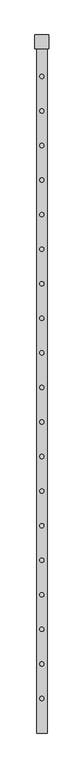
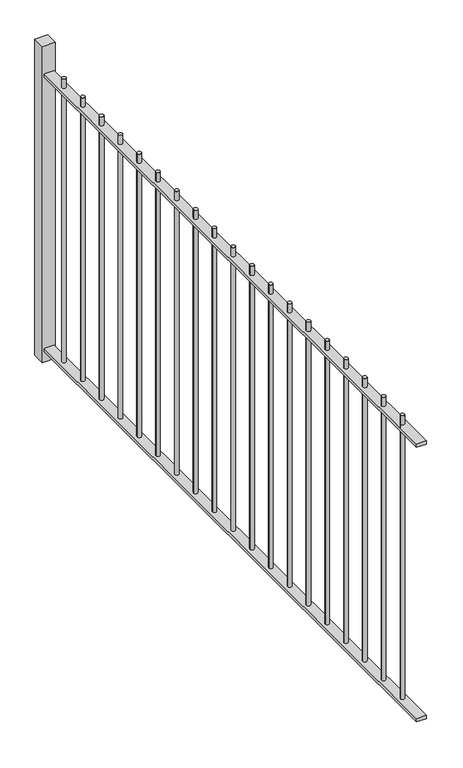
"""IFC4 building model written with IfcOpenShell, lengths in millimetres: railing geometry."""

import ifcopenshell
import ifcopenshell.guid

model = None  # the IFC model being written
_history = None  # IfcOwnerHistory: only IFC2X3 demands one
_inside = {}  # id of a spatial element -> (the spatial element, [elements in it])
_under = {}  # id of a project, library or spatial element -> (it, [spatial elements below it])
_declared = {}  # id of a project -> (the project, [libraries it declares])
_typed = {}  # id of a type object -> (the type object, [elements of that type])
_made_of = {}  # id of a material, layer set ... -> (it, [elements and type objects made of it])


def new_model(schema):
    """Start an empty IFC model of exactly this schema.

    Asked for "IFC4X3", IfcOpenShell would pick the latest addendum, in which some entities
    have other attributes; the version numbers below select the first issue.
    IFC2X3 requires an IfcOwnerHistory on every rooted entity: one is made here for all.
    """
    global model, _history
    if schema == "IFC4X3":
        model = ifcopenshell.file(schema_version=(4, 3, 0, 0))
    else:
        model = ifcopenshell.file(schema=schema)
    _inside.clear()
    _under.clear()
    _declared.clear()
    _typed.clear()
    _made_of.clear()
    _history = None
    if model.schema == "IFC2X3":
        org = make("IfcOrganization", Name="unknown")
        user = make(
            "IfcPersonAndOrganization",
            ThePerson=make("IfcPerson", FamilyName="unknown"),
            TheOrganization=org,
        )
        app = make(
            "IfcApplication",
            ApplicationDeveloper=org,
            Version="unknown",
            ApplicationFullName="unknown",
            ApplicationIdentifier="unknown",
        )
        _history = make(
            "IfcOwnerHistory",
            OwningUser=user,
            OwningApplication=app,
            ChangeAction="ADDED",
            CreationDate=0,
        )
    return model


def make(cls, **values):
    """One entity of the class cls with the attributes given. An attribute that is None is left unset."""
    return model.create_entity(
        cls, **{name: value for name, value in values.items() if value is not None}
    )


def rooted(cls, **values):
    """An entity with a GlobalId (a new one), such as an element, a storey or a relation."""
    return make(cls, GlobalId=ifcopenshell.guid.new(), OwnerHistory=_history, **values)


def si_unit(unit_type, name, prefix=None):
    """IfcSIUnit, for example si_unit("LENGTHUNIT", "METRE", prefix="MILLI")."""
    return make("IfcSIUnit", UnitType=unit_type, Prefix=prefix, Name=name)


def assignment(units):
    """IfcUnitAssignment: the units of a project."""
    return None if units is None else make("IfcUnitAssignment", Units=units)


def point(xyz):
    """IfcCartesianPoint."""
    return None if xyz is None else make("IfcCartesianPoint", Coordinates=xyz)


def direction(xyz):
    """IfcDirection."""
    return None if xyz is None else make("IfcDirection", DirectionRatios=xyz)


def frame(location, z_axis=None, x_axis=None):
    """IfcAxis2Placement3D, a coordinate frame: its origin and axes. An axis left out is left unset."""
    return make(
        "IfcAxis2Placement3D",
        Location=point(location),
        Axis=direction(z_axis),
        RefDirection=direction(x_axis),
    )


def frame_2d(location, x_axis=None):
    """IfcAxis2Placement2D, a coordinate frame in the plane: its origin and x axis."""
    return make(
        "IfcAxis2Placement2D", Location=point(location), RefDirection=direction(x_axis)
    )


def origin():
    """The frame at (0, 0, 0) with its axes left unset."""
    return frame((0.0, 0.0, 0.0))


def place(relative_to, where):
    """IfcLocalPlacement: puts the frame where relative to a parent placement (None: the world)."""
    return make(
        "IfcLocalPlacement", PlacementRelTo=relative_to, RelativePlacement=where
    )


def context(
    kind, dimensions, precision=None, world=None, true_north=None, identifier=None
):
    """IfcGeometricRepresentationContext, for example the 3D "Model" context."""
    return make(
        "IfcGeometricRepresentationContext",
        ContextIdentifier=identifier,
        ContextType=kind,
        CoordinateSpaceDimension=dimensions,
        Precision=precision,
        WorldCoordinateSystem=world,
        TrueNorth=true_north,
    )


def project(units=None, contexts=None):
    """IfcProject with its units and contexts."""
    return rooted(
        "IfcProject",
        Name="project",
        RepresentationContexts=contexts,
        UnitsInContext=assignment(units),
    )


def spatial(cls, under=None, at=None, **own):
    """A site, building, storey or space (cls), placed at a placement, below another one or the project."""
    s = rooted(cls, ObjectPlacement=at, **own)
    if under is not None:
        _under.setdefault(under.id(), (under, []))[1].append(s)
    return s


def polyline(points):
    """IfcPolyline through the points."""
    return make("IfcPolyline", Points=[point(p) for p in points])


def circle_curve(where, radius):
    """IfcCircle in the frame where."""
    return make("IfcCircle", Position=where, Radius=radius)


def trimmed(basis, trim1, trim2, sense, master):
    """IfcTrimmedCurve: the piece of a basis curve between two trims."""
    return make(
        "IfcTrimmedCurve",
        BasisCurve=basis,
        Trim1=trim1,
        Trim2=trim2,
        SenseAgreement=sense,
        MasterRepresentation=master,
    )


def segment(curve, same_sense, transition):
    """IfcCompositeCurveSegment."""
    return make(
        "IfcCompositeCurveSegment",
        Transition=transition,
        SameSense=same_sense,
        ParentCurve=curve,
    )


def composite_curve(segments, self_intersect=None):
    """IfcCompositeCurve: segments joined end to end."""
    return make("IfcCompositeCurve", Segments=segments, SelfIntersect=self_intersect)


def outline(outer, holes=None, kind="AREA"):
    """IfcArbitraryClosedProfileDef: a profile drawn as a closed curve; with holes, ...WithVoids."""
    if holes is None:
        return make("IfcArbitraryClosedProfileDef", ProfileType=kind, OuterCurve=outer)
    return make(
        "IfcArbitraryProfileDefWithVoids",
        ProfileType=kind,
        OuterCurve=outer,
        InnerCurves=holes,
    )


def extrude(swept, where, along, depth):
    """IfcExtrudedAreaSolid: the profile swept, set in the frame where, extruded along a direction by depth."""
    return make(
        "IfcExtrudedAreaSolid",
        SweptArea=swept,
        Position=where,
        ExtrudedDirection=direction(along),
        Depth=depth,
    )


def shape(context_of_items, identifier, shape_type, items):
    """IfcShapeRepresentation: the items that make up one representation, for example the "Body"."""
    return make(
        "IfcShapeRepresentation",
        ContextOfItems=context_of_items,
        RepresentationIdentifier=identifier,
        RepresentationType=shape_type,
        Items=items,
    )


def source(mapping_origin, context_of_items, identifier, shape_type, items):
    """IfcRepresentationMap: a shape defined once, which mapped items show again and again."""
    return make(
        "IfcRepresentationMap",
        MappingOrigin=mapping_origin,
        MappedRepresentation=shape(context_of_items, identifier, shape_type, items),
    )


def transform(
    local_origin,
    x_axis=None,
    y_axis=None,
    z_axis=None,
    scale=None,
    scale2=None,
    scale3=None,
    uniform=True,
):
    """IfcCartesianTransformationOperator3D, or its non-uniform kind. x_axis, y_axis, z_axis: its Axis1, 2, 3."""
    if uniform:
        return make(
            "IfcCartesianTransformationOperator3D",
            Axis1=direction(x_axis),
            Axis2=direction(y_axis),
            LocalOrigin=point(local_origin),
            Scale=scale,
            Axis3=direction(z_axis),
        )
    return make(
        "IfcCartesianTransformationOperator3DnonUniform",
        Axis1=direction(x_axis),
        Axis2=direction(y_axis),
        LocalOrigin=point(local_origin),
        Scale=scale,
        Axis3=direction(z_axis),
        Scale2=scale2,
        Scale3=scale3,
    )


def mapped(mapping_source, mapping_target):
    """IfcMappedItem: shows the shape of a source again, moved by a transform."""
    return make(
        "IfcMappedItem", MappingSource=mapping_source, MappingTarget=mapping_target
    )


def made_of(thing, what):
    """Note that an element or type object is made of a material, layer set ...; save() writes the relation."""
    if what is not None:
        _made_of.setdefault(what.id(), (what, []))[1].append(thing)
    return thing


def element(
    cls,
    number,
    at=None,
    inside=None,
    cuts=None,
    type_object=None,
    material=None,
    context=None,
    identifier="Body",
    shape_type=None,
    held_by="IfcProductDefinitionShape",
    body=None,
    shapes=None,
    **own,
):
    """One element of the class cls, such as IfcWall. Its Tag is "e" and its number.

    at: its placement. inside: the storey or other place that contains it. cuts: it is an
    opening in that element (IfcRelVoidsElement). A single representation is given by context,
    identifier, shape_type and body (its items); several are given by shapes. held_by: the class
    of the entity that holds the representations. save() writes the other relations.
    """
    e = rooted(cls, Tag="e%d" % number, ObjectPlacement=at, **own)
    if body is not None:
        shapes = [shape(context, identifier, shape_type, body)]
    if shapes is not None:
        e.Representation = make(held_by, Representations=shapes)
    if inside is not None:
        _inside.setdefault(inside.id(), (inside, []))[1].append(e)
    if cuts is not None:
        rooted(
            "IfcRelVoidsElement", RelatingBuildingElement=cuts, RelatedOpeningElement=e
        )
    if type_object is not None:
        _typed.setdefault(type_object.id(), (type_object, []))[1].append(e)
    return made_of(e, material)


def aggregate(whole, parts):
    """IfcRelAggregates: a whole, such as a stair, and the parts it consists of."""
    return rooted("IfcRelAggregates", RelatingObject=whole, RelatedObjects=parts)


def save(model, path):
    """Write the relations noted so far, then the file.

    IfcRelAggregates (storeys below a building ...), IfcRelContainedInSpatialStructure (elements
    in a storey), IfcRelDefinesByType, IfcRelAssociatesMaterial and IfcRelDeclares: one each for
    every whole, place, type object, material and project.
    """
    for whole, parts in _under.values():
        aggregate(whole, parts)
    for where, things in _inside.values():
        rooted(
            "IfcRelContainedInSpatialStructure",
            RelatedElements=things,
            RelatingStructure=where,
        )
    for kind, things in _typed.values():
        rooted("IfcRelDefinesByType", RelatedObjects=things, RelatingType=kind)
    for what, things in _made_of.values():
        rooted("IfcRelAssociatesMaterial", RelatedObjects=things, RelatingMaterial=what)
    for by, libraries in _declared.values():
        rooted("IfcRelDeclares", RelatingContext=by, RelatedDefinitions=libraries)
    model.write(path)


def railing_84141cf4(model_context):
    return source(origin(), model_context, "Body", "SweptSolid", [
        extrude(outline(polyline([(-6549.419961, 7388.8880881), (-6489.419961, 7388.8880881), (-6489.419961, 3388.8880881), (-6549.419961, 3388.8880881), (-6549.419961, 7388.8880881)])), frame((0.0, 0.0, -30.0), z_axis=(0.0, 0.0, 1.0), x_axis=(1.0, 0.0, 0.0)), (0.0, 0.0, 1.0), 20.0),
        extrude(outline(polyline([(-6549.419961, 7388.8880881), (-6489.419961, 7388.8880881), (-6489.419961, 3388.8880881), (-6549.419961, 3388.8880881), (-6549.419961, 7388.8880881)])), frame((0.0, 0.0, 1750.0), z_axis=(0.0, 0.0, 1.0), x_axis=(1.0, 0.0, 0.0)), (0.0, 0.0, 1.0), 20.0),
        extrude(outline(composite_curve([segment(trimmed(circle_curve(frame_2d((-6519.419961, 3588.8880881)), 12.5), [point((-6531.919961, 3588.8880881))], [point((-6506.919961, 3588.8880881))], False, "CARTESIAN"), True, "CONTINUOUS"), segment(trimmed(circle_curve(frame_2d((-6519.419961, 3588.8880881)), 12.5), [point((-6506.919961, 3588.8880881))], [point((-6531.919961, 3588.8880881))], False, "CARTESIAN"), True, "CONTINUOUS")], self_intersect=False)), frame((0.0, 0.0, -10.0), z_axis=(0.0, 0.0, 1.0), x_axis=(1.0, 0.0, 0.0)), (0.0, 0.0, 1.0), 1840.0),
        extrude(outline(composite_curve([segment(trimmed(circle_curve(frame_2d((-6519.419961, 3788.8880881)), 12.5), [point((-6531.919961, 3788.8880881))], [point((-6506.919961, 3788.8880881))], False, "CARTESIAN"), True, "CONTINUOUS"), segment(trimmed(circle_curve(frame_2d((-6519.419961, 3788.8880881)), 12.5), [point((-6506.919961, 3788.8880881))], [point((-6531.919961, 3788.8880881))], False, "CARTESIAN"), True, "CONTINUOUS")], self_intersect=False)), frame((0.0, 0.0, -10.0), z_axis=(0.0, 0.0, 1.0), x_axis=(1.0, 0.0, 0.0)), (0.0, 0.0, 1.0), 1840.0),
        extrude(outline(composite_curve([segment(trimmed(circle_curve(frame_2d((-6519.419961, 3988.8880881)), 12.5), [point((-6531.919961, 3988.8880881))], [point((-6506.919961, 3988.8880881))], False, "CARTESIAN"), True, "CONTINUOUS"), segment(trimmed(circle_curve(frame_2d((-6519.419961, 3988.8880881)), 12.5), [point((-6506.919961, 3988.8880881))], [point((-6531.919961, 3988.8880881))], False, "CARTESIAN"), True, "CONTINUOUS")], self_intersect=False)), frame((0.0, 0.0, -10.0), z_axis=(0.0, 0.0, 1.0), x_axis=(1.0, 0.0, 0.0)), (0.0, 0.0, 1.0), 1840.0),
        extrude(outline(composite_curve([segment(trimmed(circle_curve(frame_2d((-6519.419961, 4188.8880881)), 12.5), [point((-6531.919961, 4188.8880881))], [point((-6506.919961, 4188.8880881))], False, "CARTESIAN"), True, "CONTINUOUS"), segment(trimmed(circle_curve(frame_2d((-6519.419961, 4188.8880881)), 12.5), [point((-6506.919961, 4188.8880881))], [point((-6531.919961, 4188.8880881))], False, "CARTESIAN"), True, "CONTINUOUS")], self_intersect=False)), frame((0.0, 0.0, -10.0), z_axis=(0.0, 0.0, 1.0), x_axis=(1.0, 0.0, 0.0)), (0.0, 0.0, 1.0), 1840.0),
        extrude(outline(composite_curve([segment(trimmed(circle_curve(frame_2d((-6519.419961, 4388.8880881)), 12.5), [point((-6531.919961, 4388.8880881))], [point((-6506.919961, 4388.8880881))], False, "CARTESIAN"), True, "CONTINUOUS"), segment(trimmed(circle_curve(frame_2d((-6519.419961, 4388.8880881)), 12.5), [point((-6506.919961, 4388.8880881))], [point((-6531.919961, 4388.8880881))], False, "CARTESIAN"), True, "CONTINUOUS")], self_intersect=False)), frame((0.0, 0.0, -10.0), z_axis=(0.0, 0.0, 1.0), x_axis=(1.0, 0.0, 0.0)), (0.0, 0.0, 1.0), 1840.0),
        extrude(outline(composite_curve([segment(trimmed(circle_curve(frame_2d((-6519.419961, 4588.8880881)), 12.5), [point((-6531.919961, 4588.8880881))], [point((-6506.919961, 4588.8880881))], False, "CARTESIAN"), True, "CONTINUOUS"), segment(trimmed(circle_curve(frame_2d((-6519.419961, 4588.8880881)), 12.5), [point((-6506.919961, 4588.8880881))], [point((-6531.919961, 4588.8880881))], False, "CARTESIAN"), True, "CONTINUOUS")], self_intersect=False)), frame((0.0, 0.0, -10.0), z_axis=(0.0, 0.0, 1.0), x_axis=(1.0, 0.0, 0.0)), (0.0, 0.0, 1.0), 1840.0),
        extrude(outline(composite_curve([segment(trimmed(circle_curve(frame_2d((-6519.419961, 4788.8880881)), 12.5), [point((-6531.919961, 4788.8880881))], [point((-6506.919961, 4788.8880881))], False, "CARTESIAN"), True, "CONTINUOUS"), segment(trimmed(circle_curve(frame_2d((-6519.419961, 4788.8880881)), 12.5), [point((-6506.919961, 4788.8880881))], [point((-6531.919961, 4788.8880881))], False, "CARTESIAN"), True, "CONTINUOUS")], self_intersect=False)), frame((0.0, 0.0, -10.0), z_axis=(0.0, 0.0, 1.0), x_axis=(1.0, 0.0, 0.0)), (0.0, 0.0, 1.0), 1840.0),
        extrude(outline(composite_curve([segment(trimmed(circle_curve(frame_2d((-6519.419961, 4988.8880881)), 12.5), [point((-6531.919961, 4988.8880881))], [point((-6506.919961, 4988.8880881))], False, "CARTESIAN"), True, "CONTINUOUS"), segment(trimmed(circle_curve(frame_2d((-6519.419961, 4988.8880881)), 12.5), [point((-6506.919961, 4988.8880881))], [point((-6531.919961, 4988.8880881))], False, "CARTESIAN"), True, "CONTINUOUS")], self_intersect=False)), frame((0.0, 0.0, -10.0), z_axis=(0.0, 0.0, 1.0), x_axis=(1.0, 0.0, 0.0)), (0.0, 0.0, 1.0), 1840.0),
        extrude(outline(composite_curve([segment(trimmed(circle_curve(frame_2d((-6519.419961, 5188.8880881)), 12.5), [point((-6531.919961, 5188.8880881))], [point((-6506.919961, 5188.8880881))], False, "CARTESIAN"), True, "CONTINUOUS"), segment(trimmed(circle_curve(frame_2d((-6519.419961, 5188.8880881)), 12.5), [point((-6506.919961, 5188.8880881))], [point((-6531.919961, 5188.8880881))], False, "CARTESIAN"), True, "CONTINUOUS")], self_intersect=False)), frame((0.0, 0.0, -10.0), z_axis=(0.0, 0.0, 1.0), x_axis=(1.0, 0.0, 0.0)), (0.0, 0.0, 1.0), 1840.0),
        extrude(outline(composite_curve([segment(trimmed(circle_curve(frame_2d((-6519.419961, 5388.8880881)), 12.5), [point((-6531.919961, 5388.8880881))], [point((-6506.919961, 5388.8880881))], False, "CARTESIAN"), True, "CONTINUOUS"), segment(trimmed(circle_curve(frame_2d((-6519.419961, 5388.8880881)), 12.5), [point((-6506.919961, 5388.8880881))], [point((-6531.919961, 5388.8880881))], False, "CARTESIAN"), True, "CONTINUOUS")], self_intersect=False)), frame((0.0, 0.0, -10.0), z_axis=(0.0, 0.0, 1.0), x_axis=(1.0, 0.0, 0.0)), (0.0, 0.0, 1.0), 1840.0),
        extrude(outline(composite_curve([segment(trimmed(circle_curve(frame_2d((-6519.419961, 5588.8880881)), 12.5), [point((-6531.919961, 5588.8880881))], [point((-6506.919961, 5588.8880881))], False, "CARTESIAN"), True, "CONTINUOUS"), segment(trimmed(circle_curve(frame_2d((-6519.419961, 5588.8880881)), 12.5), [point((-6506.919961, 5588.8880881))], [point((-6531.919961, 5588.8880881))], False, "CARTESIAN"), True, "CONTINUOUS")], self_intersect=False)), frame((0.0, 0.0, -10.0), z_axis=(0.0, 0.0, 1.0), x_axis=(1.0, 0.0, 0.0)), (0.0, 0.0, 1.0), 1840.0),
        extrude(outline(composite_curve([segment(trimmed(circle_curve(frame_2d((-6519.419961, 5788.8880881)), 12.5), [point((-6531.919961, 5788.8880881))], [point((-6506.919961, 5788.8880881))], False, "CARTESIAN"), True, "CONTINUOUS"), segment(trimmed(circle_curve(frame_2d((-6519.419961, 5788.8880881)), 12.5), [point((-6506.919961, 5788.8880881))], [point((-6531.919961, 5788.8880881))], False, "CARTESIAN"), True, "CONTINUOUS")], self_intersect=False)), frame((0.0, 0.0, -10.0), z_axis=(0.0, 0.0, 1.0), x_axis=(1.0, 0.0, 0.0)), (0.0, 0.0, 1.0), 1840.0),
        extrude(outline(composite_curve([segment(trimmed(circle_curve(frame_2d((-6519.419961, 5988.8880881)), 12.5), [point((-6531.919961, 5988.8880881))], [point((-6506.919961, 5988.8880881))], False, "CARTESIAN"), True, "CONTINUOUS"), segment(trimmed(circle_curve(frame_2d((-6519.419961, 5988.8880881)), 12.5), [point((-6506.919961, 5988.8880881))], [point((-6531.919961, 5988.8880881))], False, "CARTESIAN"), True, "CONTINUOUS")], self_intersect=False)), frame((0.0, 0.0, -10.0), z_axis=(0.0, 0.0, 1.0), x_axis=(1.0, 0.0, 0.0)), (0.0, 0.0, 1.0), 1840.0),
        extrude(outline(composite_curve([segment(trimmed(circle_curve(frame_2d((-6519.419961, 6188.8880881)), 12.5), [point((-6531.919961, 6188.8880881))], [point((-6506.919961, 6188.8880881))], False, "CARTESIAN"), True, "CONTINUOUS"), segment(trimmed(circle_curve(frame_2d((-6519.419961, 6188.8880881)), 12.5), [point((-6506.919961, 6188.8880881))], [point((-6531.919961, 6188.8880881))], False, "CARTESIAN"), True, "CONTINUOUS")], self_intersect=False)), frame((0.0, 0.0, -10.0), z_axis=(0.0, 0.0, 1.0), x_axis=(1.0, 0.0, 0.0)), (0.0, 0.0, 1.0), 1840.0),
        extrude(outline(composite_curve([segment(trimmed(circle_curve(frame_2d((-6519.419961, 6388.8880881)), 12.5), [point((-6531.919961, 6388.8880881))], [point((-6506.919961, 6388.8880881))], False, "CARTESIAN"), True, "CONTINUOUS"), segment(trimmed(circle_curve(frame_2d((-6519.419961, 6388.8880881)), 12.5), [point((-6506.919961, 6388.8880881))], [point((-6531.919961, 6388.8880881))], False, "CARTESIAN"), True, "CONTINUOUS")], self_intersect=False)), frame((0.0, 0.0, -10.0), z_axis=(0.0, 0.0, 1.0), x_axis=(1.0, 0.0, 0.0)), (0.0, 0.0, 1.0), 1840.0),
        extrude(outline(composite_curve([segment(trimmed(circle_curve(frame_2d((-6519.419961, 6588.8880881)), 12.5), [point((-6531.919961, 6588.8880881))], [point((-6506.919961, 6588.8880881))], False, "CARTESIAN"), True, "CONTINUOUS"), segment(trimmed(circle_curve(frame_2d((-6519.419961, 6588.8880881)), 12.5), [point((-6506.919961, 6588.8880881))], [point((-6531.919961, 6588.8880881))], False, "CARTESIAN"), True, "CONTINUOUS")], self_intersect=False)), frame((0.0, 0.0, -10.0), z_axis=(0.0, 0.0, 1.0), x_axis=(1.0, 0.0, 0.0)), (0.0, 0.0, 1.0), 1840.0),
        extrude(outline(composite_curve([segment(trimmed(circle_curve(frame_2d((-6519.419961, 6788.8880881)), 12.5), [point((-6531.919961, 6788.8880881))], [point((-6506.919961, 6788.8880881))], False, "CARTESIAN"), True, "CONTINUOUS"), segment(trimmed(circle_curve(frame_2d((-6519.419961, 6788.8880881)), 12.5), [point((-6506.919961, 6788.8880881))], [point((-6531.919961, 6788.8880881))], False, "CARTESIAN"), True, "CONTINUOUS")], self_intersect=False)), frame((0.0, 0.0, -10.0), z_axis=(0.0, 0.0, 1.0), x_axis=(1.0, 0.0, 0.0)), (0.0, 0.0, 1.0), 1840.0),
        extrude(outline(composite_curve([segment(trimmed(circle_curve(frame_2d((-6519.419961, 6988.8880881)), 12.5), [point((-6531.919961, 6988.8880881))], [point((-6506.919961, 6988.8880881))], False, "CARTESIAN"), True, "CONTINUOUS"), segment(trimmed(circle_curve(frame_2d((-6519.419961, 6988.8880881)), 12.5), [point((-6506.919961, 6988.8880881))], [point((-6531.919961, 6988.8880881))], False, "CARTESIAN"), True, "CONTINUOUS")], self_intersect=False)), frame((0.0, 0.0, -10.0), z_axis=(0.0, 0.0, 1.0), x_axis=(1.0, 0.0, 0.0)), (0.0, 0.0, 1.0), 1840.0),
        extrude(outline(composite_curve([segment(trimmed(circle_curve(frame_2d((-6519.419961, 7188.8880881)), 12.5), [point((-6531.919961, 7188.8880881))], [point((-6506.919961, 7188.8880881))], False, "CARTESIAN"), True, "CONTINUOUS"), segment(trimmed(circle_curve(frame_2d((-6519.419961, 7188.8880881)), 12.5), [point((-6506.919961, 7188.8880881))], [point((-6531.919961, 7188.8880881))], False, "CARTESIAN"), True, "CONTINUOUS")], self_intersect=False)), frame((0.0, 0.0, -10.0), z_axis=(0.0, 0.0, 1.0), x_axis=(1.0, 0.0, 0.0)), (0.0, 0.0, 1.0), 1840.0),
        extrude(outline(polyline([(-6479.419961, 7428.8880881), (-6479.419961, 7348.8880881), (-6559.419961, 7348.8880881), (-6559.419961, 7428.8880881), (-6479.419961, 7428.8880881)])), frame((0.0, 0.0, -100.0), z_axis=(0.0, 0.0, 1.0), x_axis=(1.0, 0.0, 0.0)), (0.0, 0.0, 1.0), 2050.0),
    ])


if __name__ == "__main__":
    model = new_model("IFC4")
    model_context = context("Model", 3, world=origin())
    ifc_project = project(units=[si_unit("LENGTHUNIT", "METRE", prefix="MILLI")], contexts=[model_context])
    site = spatial("IfcSite", under=ifc_project)
    building = spatial("IfcBuilding", under=site)
    placement = place(None, origin())
    railing_shape = railing_84141cf4(model_context)
    element("IfcRailing", 1, at=placement, inside=building, context=model_context, shape_type="MappedRepresentation", body=[
        mapped(railing_shape, transform((0.0, 0.0, 0.0), x_axis=(1.0, 0.0, 0.0), y_axis=(0.0, 1.0, 0.0), z_axis=(0.0, 0.0, 1.0))),
    ])
    save(model, "model.ifc")

# Revit data of these elements
# Element 1 (IfcRailing)
#   Materials on its faces: "NLRS_h2_staal_generiek zwart_gen_rsf", "NLRS_h2_staal_gen_rsf"
# Materials
#   "NLRS_h2_staal_generiek zwart_gen_rsf": class "Metal", colour RGB 189 187 185, transparency 0, Manufacturer = "RevitGG", URL = "www.revitgg.nl", Description = "Staal, generiek materiaal", Cost = 0
#   "NLRS_h2_staal_gen_rsf": class "H - Metaal", colour RGB 189 187 185, transparency 0, Keynote = "h2", Model = "generiek", Manufacturer = "Revit Standards Foundation", URL = "www.revitstandards.org", Description = "staal", Cost = 0
